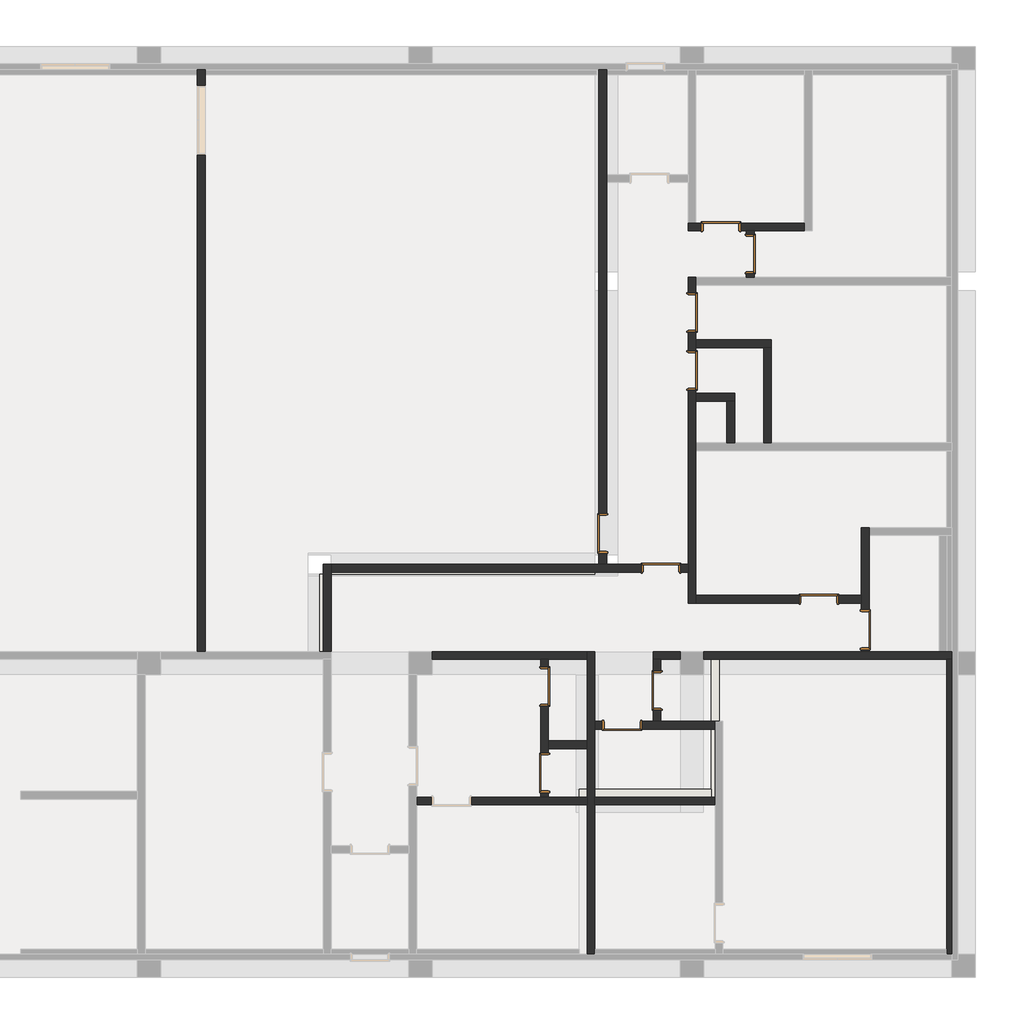
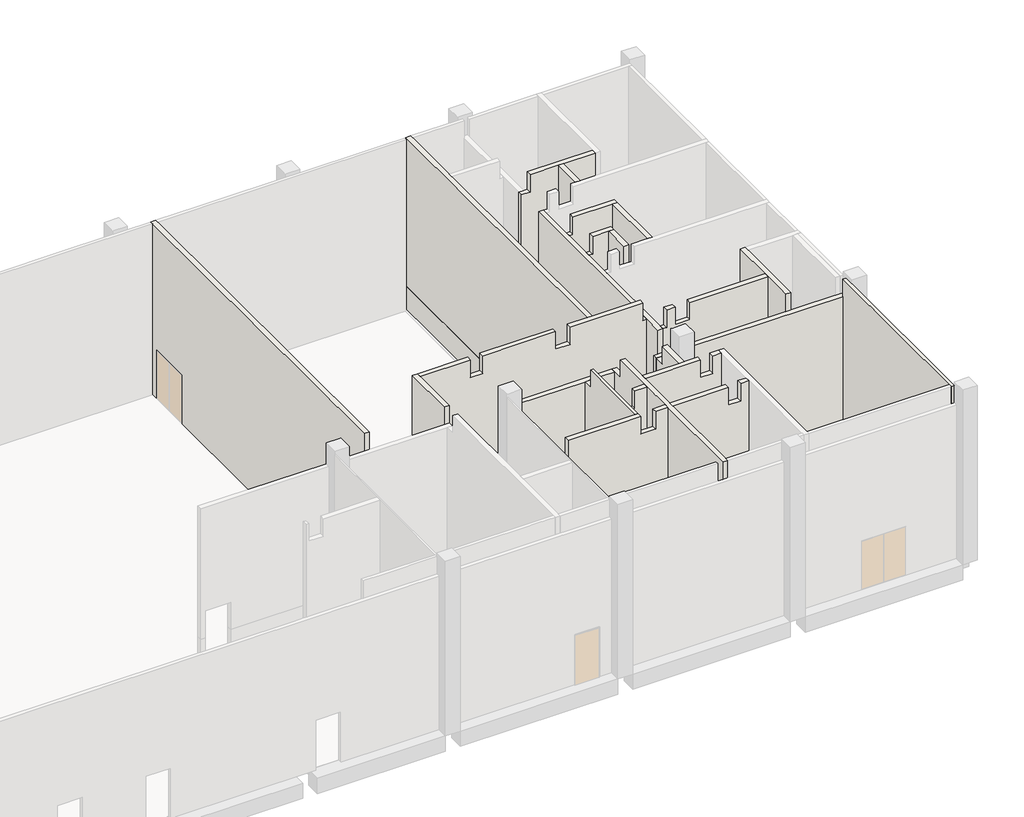
# One storey, part 2 of 4: 29 walls, 12 doors.
"""IFC4 building model written with IfcOpenShell, lengths in millimetres."""

import ifcopenshell
import ifcopenshell.guid

model = None  # the IFC model being written
_history = None  # IfcOwnerHistory: only IFC2X3 demands one
_inside = {}  # id of a spatial element -> (the spatial element, [elements in it])
_under = {}  # id of a project, library or spatial element -> (it, [spatial elements below it])
_declared = {}  # id of a project -> (the project, [libraries it declares])
_typed = {}  # id of a type object -> (the type object, [elements of that type])
_made_of = {}  # id of a material, layer set ... -> (it, [elements and type objects made of it])


def new_model(schema):
    """Start an empty IFC model of exactly this schema.

    Asked for "IFC4X3", IfcOpenShell would pick the latest addendum, in which some entities
    have other attributes; the version numbers below select the first issue.
    IFC2X3 requires an IfcOwnerHistory on every rooted entity: one is made here for all.
    """
    global model, _history
    if schema == "IFC4X3":
        model = ifcopenshell.file(schema_version=(4, 3, 0, 0))
    else:
        model = ifcopenshell.file(schema=schema)
    _inside.clear()
    _under.clear()
    _declared.clear()
    _typed.clear()
    _made_of.clear()
    _history = None
    if model.schema == "IFC2X3":
        org = make("IfcOrganization", Name="unknown")
        user = make(
            "IfcPersonAndOrganization",
            ThePerson=make("IfcPerson", FamilyName="unknown"),
            TheOrganization=org,
        )
        app = make(
            "IfcApplication",
            ApplicationDeveloper=org,
            Version="unknown",
            ApplicationFullName="unknown",
            ApplicationIdentifier="unknown",
        )
        _history = make(
            "IfcOwnerHistory",
            OwningUser=user,
            OwningApplication=app,
            ChangeAction="ADDED",
            CreationDate=0,
        )
    return model


def make(cls, **values):
    """One entity of the class cls with the attributes given. An attribute that is None is left unset."""
    return model.create_entity(
        cls, **{name: value for name, value in values.items() if value is not None}
    )


def rooted(cls, **values):
    """An entity with a GlobalId (a new one), such as an element, a storey or a relation."""
    return make(cls, GlobalId=ifcopenshell.guid.new(), OwnerHistory=_history, **values)


def si_unit(unit_type, name, prefix=None):
    """IfcSIUnit, for example si_unit("LENGTHUNIT", "METRE", prefix="MILLI")."""
    return make("IfcSIUnit", UnitType=unit_type, Prefix=prefix, Name=name)


def assignment(units):
    """IfcUnitAssignment: the units of a project."""
    return None if units is None else make("IfcUnitAssignment", Units=units)


def point(xyz):
    """IfcCartesianPoint."""
    return None if xyz is None else make("IfcCartesianPoint", Coordinates=xyz)


def direction(xyz):
    """IfcDirection."""
    return None if xyz is None else make("IfcDirection", DirectionRatios=xyz)


def frame(location, z_axis=None, x_axis=None):
    """IfcAxis2Placement3D, a coordinate frame: its origin and axes. An axis left out is left unset."""
    return make(
        "IfcAxis2Placement3D",
        Location=point(location),
        Axis=direction(z_axis),
        RefDirection=direction(x_axis),
    )


def origin():
    """The frame at (0, 0, 0) with its axes left unset."""
    return frame((0.0, 0.0, 0.0))


def origin_with_axes():
    """The frame at (0, 0, 0) with the z axis (0, 0, 1) and the x axis (1, 0, 0) written out."""
    return frame((0.0, 0.0, 0.0), z_axis=(0.0, 0.0, 1.0), x_axis=(1.0, 0.0, 0.0))


def place(relative_to, where):
    """IfcLocalPlacement: puts the frame where relative to a parent placement (None: the world)."""
    return make(
        "IfcLocalPlacement", PlacementRelTo=relative_to, RelativePlacement=where
    )


def context(
    kind, dimensions, precision=None, world=None, true_north=None, identifier=None
):
    """IfcGeometricRepresentationContext, for example the 3D "Model" context."""
    return make(
        "IfcGeometricRepresentationContext",
        ContextIdentifier=identifier,
        ContextType=kind,
        CoordinateSpaceDimension=dimensions,
        Precision=precision,
        WorldCoordinateSystem=world,
        TrueNorth=true_north,
    )


def project(units=None, contexts=None):
    """IfcProject with its units and contexts."""
    return rooted(
        "IfcProject",
        Name="project",
        RepresentationContexts=contexts,
        UnitsInContext=assignment(units),
    )


def spatial(cls, under=None, at=None, **own):
    """A site, building, storey or space (cls), placed at a placement, below another one or the project."""
    s = rooted(cls, ObjectPlacement=at, **own)
    if under is not None:
        _under.setdefault(under.id(), (under, []))[1].append(s)
    return s


def polyline(points):
    """IfcPolyline through the points."""
    return make("IfcPolyline", Points=[point(p) for p in points])


def outline(outer, holes=None, kind="AREA"):
    """IfcArbitraryClosedProfileDef: a profile drawn as a closed curve; with holes, ...WithVoids."""
    if holes is None:
        return make("IfcArbitraryClosedProfileDef", ProfileType=kind, OuterCurve=outer)
    return make(
        "IfcArbitraryProfileDefWithVoids",
        ProfileType=kind,
        OuterCurve=outer,
        InnerCurves=holes,
    )


def extrude(swept, where, along, depth):
    """IfcExtrudedAreaSolid: the profile swept, set in the frame where, extruded along a direction by depth."""
    return make(
        "IfcExtrudedAreaSolid",
        SweptArea=swept,
        Position=where,
        ExtrudedDirection=direction(along),
        Depth=depth,
    )


def faces_of(points, faces, orient=None, outer=None):
    """IfcFace entities. A face is a list of loops; a loop is a list of indices into points, from 0.

    orient and outer hold one flag for each loop. By default every Orientation is true, the
    first loop of a face is its IfcFaceOuterBound and the others are IfcFaceBound.
    """
    made = []
    for i, loops in enumerate(faces):
        bounds = []
        for j, loop in enumerate(loops):
            is_outer = j == 0 if outer is None else outer[i][j]
            bounds.append(
                make(
                    "IfcFaceOuterBound" if is_outer else "IfcFaceBound",
                    Bound=make("IfcPolyLoop", Polygon=[points[k] for k in loop]),
                    Orientation=True if orient is None else orient[i][j],
                )
            )
        made.append(make("IfcFace", Bounds=bounds))
    return made


def faceted_brep(points, faces, orient=None, outer=None, voids=None):
    """IfcFacetedBrep: a solid bounded by flat faces; with voids (closed shells), ...WithVoids."""
    shared = [point(p) for p in points]
    hull = make("IfcClosedShell", CfsFaces=faces_of(shared, faces, orient, outer))
    if voids is None:
        return make("IfcFacetedBrep", Outer=hull)
    return make(
        "IfcFacetedBrepWithVoids",
        Outer=hull,
        Voids=[
            make(cls, CfsFaces=faces_of(shared, fs, o, b)) for cls, fs, o, b in voids
        ],
    )


def shape(context_of_items, identifier, shape_type, items):
    """IfcShapeRepresentation: the items that make up one representation, for example the "Body"."""
    return make(
        "IfcShapeRepresentation",
        ContextOfItems=context_of_items,
        RepresentationIdentifier=identifier,
        RepresentationType=shape_type,
        Items=items,
    )


def source(mapping_origin, context_of_items, identifier, shape_type, items):
    """IfcRepresentationMap: a shape defined once, which mapped items show again and again."""
    return make(
        "IfcRepresentationMap",
        MappingOrigin=mapping_origin,
        MappedRepresentation=shape(context_of_items, identifier, shape_type, items),
    )


def transform(
    local_origin,
    x_axis=None,
    y_axis=None,
    z_axis=None,
    scale=None,
    scale2=None,
    scale3=None,
    uniform=True,
):
    """IfcCartesianTransformationOperator3D, or its non-uniform kind. x_axis, y_axis, z_axis: its Axis1, 2, 3."""
    if uniform:
        return make(
            "IfcCartesianTransformationOperator3D",
            Axis1=direction(x_axis),
            Axis2=direction(y_axis),
            LocalOrigin=point(local_origin),
            Scale=scale,
            Axis3=direction(z_axis),
        )
    return make(
        "IfcCartesianTransformationOperator3DnonUniform",
        Axis1=direction(x_axis),
        Axis2=direction(y_axis),
        LocalOrigin=point(local_origin),
        Scale=scale,
        Axis3=direction(z_axis),
        Scale2=scale2,
        Scale3=scale3,
    )


def mapped(mapping_source, mapping_target):
    """IfcMappedItem: shows the shape of a source again, moved by a transform."""
    return make(
        "IfcMappedItem", MappingSource=mapping_source, MappingTarget=mapping_target
    )


def made_of(thing, what):
    """Note that an element or type object is made of a material, layer set ...; save() writes the relation."""
    if what is not None:
        _made_of.setdefault(what.id(), (what, []))[1].append(thing)
    return thing


def element(
    cls,
    number,
    at=None,
    inside=None,
    cuts=None,
    type_object=None,
    material=None,
    context=None,
    identifier="Body",
    shape_type=None,
    held_by="IfcProductDefinitionShape",
    body=None,
    shapes=None,
    **own,
):
    """One element of the class cls, such as IfcWall. Its Tag is "e" and its number.

    at: its placement. inside: the storey or other place that contains it. cuts: it is an
    opening in that element (IfcRelVoidsElement). A single representation is given by context,
    identifier, shape_type and body (its items); several are given by shapes. held_by: the class
    of the entity that holds the representations. save() writes the other relations.
    """
    e = rooted(cls, Tag="e%d" % number, ObjectPlacement=at, **own)
    if body is not None:
        shapes = [shape(context, identifier, shape_type, body)]
    if shapes is not None:
        e.Representation = make(held_by, Representations=shapes)
    if inside is not None:
        _inside.setdefault(inside.id(), (inside, []))[1].append(e)
    if cuts is not None:
        rooted(
            "IfcRelVoidsElement", RelatingBuildingElement=cuts, RelatedOpeningElement=e
        )
    if type_object is not None:
        _typed.setdefault(type_object.id(), (type_object, []))[1].append(e)
    return made_of(e, material)


def aggregate(whole, parts):
    """IfcRelAggregates: a whole, such as a stair, and the parts it consists of."""
    return rooted("IfcRelAggregates", RelatingObject=whole, RelatedObjects=parts)


def save(model, path):
    """Write the relations noted so far, then the file.

    IfcRelAggregates (storeys below a building ...), IfcRelContainedInSpatialStructure (elements
    in a storey), IfcRelDefinesByType, IfcRelAssociatesMaterial and IfcRelDeclares: one each for
    every whole, place, type object, material and project.
    """
    for whole, parts in _under.values():
        aggregate(whole, parts)
    for where, things in _inside.values():
        rooted(
            "IfcRelContainedInSpatialStructure",
            RelatedElements=things,
            RelatingStructure=where,
        )
    for kind, things in _typed.values():
        rooted("IfcRelDefinesByType", RelatedObjects=things, RelatingType=kind)
    for what, things in _made_of.values():
        rooted("IfcRelAssociatesMaterial", RelatedObjects=things, RelatingMaterial=what)
    for by, libraries in _declared.values():
        rooted("IfcRelDeclares", RelatingContext=by, RelatedDefinitions=libraries)
    model.write(path)


def single_door_steel_f73fbc53(model_context):
    return source(origin(), model_context, "Body", "SolidModel", [
        extrude(outline(polyline([(480.0, -130.0), (-480.0, -130.0), (-480.0, -95.0), (480.0, -95.0), (480.0, -130.0)])), origin_with_axes(), (0.0, 0.0, 1.0), 2130.0),
        faceted_brep([(480.0, -130.0, 0.0), (480.0, -95.0, 0.0), (460.0, -95.0, 0.0), (460.0, 95.0, 0.0), (480.0, 95.0, 0.0), (480.0, 130.0, 0.0), (510.0, 130.0, 0.0), (510.0, -130.0, 0.0), (510.0, -130.0, 2160.0), (-510.0, -130.0, 2160.0), (-510.0, -130.0, 0.0), (-480.0, -130.0, 0.0), (-480.0, -130.0, 2130.0), (480.0, -130.0, 2130.0), (510.0, 130.0, 2160.0), (480.0, 130.0, 2130.0), (-480.0, 130.0, 2130.0), (-480.0, 130.0, 0.0), (-510.0, 130.0, 0.0), (-510.0, 130.0, 2160.0), (480.0, 95.0, 2130.0), (460.0, 95.0, 2110.0), (-460.0, 95.0, 2110.0), (-460.0, 95.0, 0.0), (-480.0, 95.0, 0.0), (-480.0, 95.0, 2130.0), (460.0, -95.0, 2110.0), (480.0, -95.0, 2130.0), (-480.0, -95.0, 2130.0), (-480.0, -95.0, 0.0), (-460.0, -95.0, 0.0), (-460.0, -95.0, 2110.0)], [[[0, 1, 2, 3, 4, 5, 6, 7]], [[7, 8, 9, 10, 11, 12, 13, 0]], [[6, 14, 8, 7]], [[5, 15, 16, 17, 18, 19, 14, 6]], [[4, 20, 15, 5]], [[3, 21, 22, 23, 24, 25, 20, 4]], [[2, 26, 21, 3]], [[1, 27, 28, 29, 30, 31, 26, 2]], [[0, 13, 27, 1]], [[12, 11, 29, 28]], [[11, 10, 18, 17, 24, 23, 30, 29]], [[19, 18, 10, 9]], [[25, 24, 17, 16]], [[31, 30, 23, 22]], [[14, 19, 9, 8]], [[20, 25, 16, 15]], [[26, 31, 22, 21]], [[13, 12, 28, 27]]]),
    ])


def single_door_steel_4bf023c6(model_context):
    return source(origin(), model_context, "Body", "SolidModel", [
        extrude(outline(polyline([(480.0, 130.0), (480.0, 95.0), (-480.0, 95.0), (-480.0, 130.0), (480.0, 130.0)])), origin_with_axes(), (0.0, 0.0, 1.0), 2130.0),
        faceted_brep([(480.0, 130.0, 0.0), (510.0, 130.0, 0.0), (510.0, -130.0, 0.0), (480.0, -130.0, 0.0), (480.0, -95.0, 0.0), (460.0, -95.0, 0.0), (460.0, 95.0, 0.0), (480.0, 95.0, 0.0), (480.0, 130.0, 2130.0), (-480.0, 130.0, 2130.0), (-480.0, 130.0, 0.0), (-510.0, 130.0, 0.0), (-510.0, 130.0, 2160.0), (510.0, 130.0, 2160.0), (510.0, -130.0, 2160.0), (-510.0, -130.0, 2160.0), (-510.0, -130.0, 0.0), (-480.0, -130.0, 0.0), (-480.0, -130.0, 2130.0), (480.0, -130.0, 2130.0), (480.0, -95.0, 2130.0), (-480.0, -95.0, 2130.0), (-480.0, -95.0, 0.0), (-460.0, -95.0, 0.0), (-460.0, -95.0, 2110.0), (460.0, -95.0, 2110.0), (460.0, 95.0, 2110.0), (-460.0, 95.0, 2110.0), (-460.0, 95.0, 0.0), (-480.0, 95.0, 0.0), (-480.0, 95.0, 2130.0), (480.0, 95.0, 2130.0)], [[[0, 1, 2, 3, 4, 5, 6, 7]], [[1, 0, 8, 9, 10, 11, 12, 13]], [[2, 1, 13, 14]], [[3, 2, 14, 15, 16, 17, 18, 19]], [[4, 3, 19, 20]], [[5, 4, 20, 21, 22, 23, 24, 25]], [[6, 5, 25, 26]], [[7, 6, 26, 27, 28, 29, 30, 31]], [[0, 7, 31, 8]], [[9, 30, 29, 10]], [[10, 29, 28, 23, 22, 17, 16, 11]], [[15, 12, 11, 16]], [[21, 18, 17, 22]], [[27, 24, 23, 28]], [[14, 13, 12, 15]], [[20, 19, 18, 21]], [[26, 25, 24, 27]], [[8, 31, 30, 9]]]),
    ])


model = new_model("IFC4")

# Units and contexts
model_context = context("Model", 3, world=origin())
ifc_project = project(units=[si_unit("LENGTHUNIT", "METRE", prefix="MILLI")], contexts=[model_context])

# Site, building, storey
site = spatial("IfcSite", under=ifc_project)
building = spatial("IfcBuilding", under=site)
storey = spatial("IfcBuildingStorey", under=building, Name="TOC(GF)", Elevation=97049.9618634)

# Doors
placement = place(None, origin())
single_door_steel_shape = single_door_steel_f73fbc53(model_context)
element("IfcDoor", 1, ObjectType="Single Door_Steel : H_DR_AR B12_Door_Single FSD 01", at=placement, inside=storey, context=model_context, shape_type="MappedRepresentation", body=[
    mapped(single_door_steel_shape, transform((47500.0, -1150.0, 97049.9618634), x_axis=(0.0, 1.0, 0.0), y_axis=(-1.0, 0.0, 0.0), z_axis=(0.0, 0.0, 1.0))),
])
element("IfcDoor", 2, ObjectType="Single Door_Steel : H_DR_AR B12_Door_Single FSD 01", at=placement, inside=storey, context=model_context, shape_type="MappedRepresentation", body=[
    mapped(single_door_steel_shape, transform((45200.0, -9250.0, 97049.9618634), x_axis=(-1.0, 0.0, 0.0), y_axis=(0.0, -1.0, 0.0), z_axis=(0.0, 0.0, 1.0))),
])
element("IfcDoor", 3, ObjectType="Single Door_Steel : H_DR_AR B12_Door_Single FSD 01", at=placement, inside=storey, context=model_context, shape_type="MappedRepresentation", body=[
    mapped(single_door_steel_shape, transform((50470.0, -10836.4720793, 97049.9618634), x_axis=(0.0, 1.0, 0.0), y_axis=(-1.0, 0.0, 0.0), z_axis=(0.0, 0.0, 1.0))),
])
element("IfcDoor", 4, ObjectType="Single Door_Steel : H_DR_AR B12_Door_Single FSD 01", at=placement, inside=storey, context=model_context, shape_type="MappedRepresentation", body=[
    mapped(single_door_steel_shape, transform((44201.4300122, -13300.0, 97049.9618634), x_axis=(1.0, 0.0, 0.0), y_axis=(0.0, 1.0, 0.0), z_axis=(0.0, 0.0, 1.0))),
])
single_door_steel_2_shape = single_door_steel_4bf023c6(model_context)
element("IfcDoor", 5, ObjectType="Single Door_Steel : H_DR_AR B12_Door_Single FSD 01", at=placement, inside=storey, context=model_context, shape_type="MappedRepresentation", body=[
    mapped(single_door_steel_2_shape, transform((46750.0, -450.0, 97049.9618634), x_axis=(1.0, 0.0, 0.0), y_axis=(0.0, 1.0, 0.0), z_axis=(0.0, 0.0, 1.0))),
])
element("IfcDoor", 6, ObjectType="Single Door_Steel : H_DR_AR B12_Door_Single FSD 01", at=placement, inside=storey, context=model_context, shape_type="MappedRepresentation", body=[
    mapped(single_door_steel_2_shape, transform((46000.0, -2657.5, 97049.9618634), x_axis=(0.0, -1.0, 0.0), y_axis=(1.0, 0.0, 0.0), z_axis=(0.0, 0.0, 1.0))),
])
element("IfcDoor", 7, ObjectType="Single Door_Steel : H_DR_AR B12_Door_Single FSD 01", at=placement, inside=storey, context=model_context, shape_type="MappedRepresentation", body=[
    mapped(single_door_steel_2_shape, transform((46000.0, -4155.0, 97049.9618634), x_axis=(0.0, -1.0, 0.0), y_axis=(1.0, 0.0, 0.0), z_axis=(0.0, 0.0, 1.0))),
])
element("IfcDoor", 8, ObjectType="Single Door_Steel : H_DR_AR B12_Door_Single FSD 01", at=placement, inside=storey, context=model_context, shape_type="MappedRepresentation", body=[
    mapped(single_door_steel_2_shape, transform((43700.0, -8350.0, 97049.9618634), x_axis=(0.0, 1.0, 0.0), y_axis=(-1.0, 0.0, 0.0), z_axis=(0.0, 0.0, 1.0))),
])
element("IfcDoor", 9, ObjectType="Single Door_Steel : H_DR_AR B12_Door_Single FSD 01", at=placement, inside=storey, context=model_context, shape_type="MappedRepresentation", body=[
    mapped(single_door_steel_2_shape, transform((49270.0, -10050.0, 97049.9618634), x_axis=(1.0, 0.0, 0.0), y_axis=(0.0, 1.0, 0.0), z_axis=(0.0, 0.0, 1.0))),
])
element("IfcDoor", 10, ObjectType="Single Door_Steel : H_DR_AR B12_Door_Single FSD 01", at=placement, inside=storey, context=model_context, shape_type="MappedRepresentation", body=[
    mapped(single_door_steel_2_shape, transform((45100.0, -12400.0, 97049.9618634), x_axis=(0.0, 1.0, 0.0), y_axis=(-1.0, 0.0, 0.0), z_axis=(0.0, 0.0, 1.0))),
])
element("IfcDoor", 11, ObjectType="Single Door_Steel : H_DR_AR B12_Door_Single FSD 01", at=placement, inside=storey, context=model_context, shape_type="MappedRepresentation", body=[
    mapped(single_door_steel_2_shape, transform((42200.0, -12300.0, 97049.9618634), x_axis=(0.0, -1.0, 0.0), y_axis=(1.0, 0.0, 0.0), z_axis=(0.0, 0.0, 1.0))),
])
element("IfcDoor", 12, ObjectType="Single Door_Steel : H_DR_AR B12_Door_Single FSD 01", at=placement, inside=storey, context=model_context, shape_type="MappedRepresentation", body=[
    mapped(single_door_steel_2_shape, transform((42200.0, -14524.618743, 97049.9618634), x_axis=(0.0, 1.0, 0.0), y_axis=(-1.0, 0.0, 0.0), z_axis=(0.0, 0.0, 1.0))),
])

# Walls
element("IfcWall", 13, ObjectType="H_WA_AR_B02_Ext Wall_RC_T200_W2", at=placement, inside=storey, context=model_context, shape_type="Brep", body=[
    faceted_brep([(36700.0, -9200.0, 97049.9618634), (36700.0, -9200.0, 98049.9618634), (43500.0, -9200.0, 98049.9618634), (43500.0, -9200.0, 97049.9618634), (36700.0, -9400.0, 98049.9618634), (36700.0, -9400.0, 97049.9618634), (43500.0, -9400.0, 97049.9618634), (43500.0, -9400.0, 98049.9618634), (36700.0, -9350.0, 98049.9618634)], [[[0, 1, 2, 3]], [[4, 5, 6, 7]], [[5, 0, 3, 6]], [[1, 8, 4, 7, 2]], [[1, 0, 5, 4, 8]], [[3, 2, 7, 6]]]),
])
element("IfcWall", 14, ObjectType="H_WA_AR_B02_Ext Wall_RC_T200_W2", at=placement, inside=storey, context=model_context, shape_type="Brep", body=[
    faceted_brep([(36400.0, -9400.0, 97049.9618634), (36400.0, -11400.0, 97049.9618634), (36400.0, -11600.0, 97049.9618634), (36400.0, -11600.0, 98049.9618634), (36400.0, -11400.0, 98049.9618634), (36400.0, -9400.0, 98049.9618634), (36600.0, -9400.0, 97049.9618634), (36600.0, -9400.0, 98049.9618634), (36600.0, -11400.0, 98049.9618634), (36600.0, -11600.0, 98049.9618634), (36600.0, -11600.0, 97049.9618634), (36600.0, -11400.0, 97049.9618634), (36500.0, -11600.0, 97049.9618634)], [[[0, 1, 2, 3, 4, 5]], [[6, 7, 8, 9, 10, 11]], [[2, 1, 0, 6, 11, 10, 12]], [[5, 4, 3, 9, 8, 7]], [[0, 5, 7, 6]], [[3, 2, 12, 10, 9]]]),
])
element("IfcWall", 15, ObjectType="H_WA_AR_B02_Ext Wall_RC_T200_W2", at=placement, inside=storey, context=model_context, shape_type="Brep", body=[
    faceted_brep([(43800.0, -8900.0, 98049.9618634), (43800.0, -8900.0, 97049.9618634), (43800.0, -8860.0, 97049.9618634), (43800.0, -8860.0, 98049.9618634), (43600.0, -8900.0, 97049.9618634), (43600.0, -8900.0, 98049.9618634), (43600.0, -8860.0, 98049.9618634), (43600.0, -8860.0, 97049.9618634)], [[[0, 1, 2, 3]], [[4, 5, 6, 7]], [[1, 4, 7, 2]], [[5, 0, 3, 6]], [[1, 0, 5, 4]], [[3, 2, 7, 6]]]),
    faceted_brep([(43800.0, -7840.0, 98049.9618634), (43800.0, -7840.0, 97049.9618634), (43800.0, -2100.0, 97049.9618634), (43800.0, -2100.0, 98049.9618634), (43600.0, -7840.0, 97049.9618634), (43600.0, -7840.0, 98049.9618634), (43600.0, -2100.0, 98049.9618634), (43600.0, -2100.0, 97049.9618634)], [[[0, 1, 2, 3]], [[4, 5, 6, 7]], [[1, 4, 7, 2]], [[5, 0, 3, 6]], [[3, 2, 7, 6]], [[1, 0, 5, 4]]]),
    faceted_brep([(43800.0, 3600.0, 97049.9618634), (43800.0, 3600.0, 98049.9618634), (43800.0, -1600.0, 98049.9618634), (43800.0, -1600.0, 97049.9618634), (43800.0, 700.0, 97049.9618634), (43800.0, 900.0, 97049.9618634), (43800.0, 3474.0, 97049.9618634), (43600.0, 3600.0, 98049.9618634), (43600.0, 3600.0, 97049.9618634), (43600.0, -1600.0, 97049.9618634), (43600.0, -1600.0, 98049.9618634)], [[[0, 1, 2, 3, 4, 5, 6]], [[7, 8, 9, 10]], [[8, 0, 6, 5, 4, 3, 9]], [[1, 7, 10, 2]], [[1, 0, 8, 7]], [[3, 2, 10, 9]]]),
])
element("IfcWall", 16, ObjectType="H_WA_AR_B02_Ext Wall_RC_T200_W2", at=placement, inside=storey, context=model_context, shape_type="Brep", body=[
    faceted_brep([(46300.0, -11600.0, 97049.9618634), (46500.0, -11600.0, 97049.9618634), (46700.0, -11600.0, 97049.9618634), (52574.0, -11600.0, 97049.9618634), (52700.0, -11600.0, 97049.9618634), (52700.0, -11600.0, 98049.9618634), (52574.0, -11600.0, 98049.9618634), (46700.0, -11600.0, 98049.9618634), (46500.0, -11600.0, 98049.9618634), (46300.0, -11600.0, 98049.9618634), (46300.0, -11400.0, 97049.9618634), (46300.0, -11400.0, 98049.9618634), (52574.0, -11400.0, 98049.9618634), (52700.0, -11400.0, 98049.9618634), (52700.0, -11400.0, 97049.9618634), (52574.0, -11400.0, 97049.9618634), (52374.0, -11400.0, 97049.9618634), (50570.0, -11400.0, 97049.9618634), (50370.0, -11400.0, 97049.9618634)], [[[0, 1, 2, 3, 4, 5, 6, 7, 8, 9]], [[10, 11, 12, 13, 14, 15, 16, 17, 18]], [[4, 3, 2, 1, 0, 10, 18, 17, 16, 15, 14]], [[9, 8, 7, 6, 5, 13, 12, 11]], [[0, 9, 11, 10]], [[5, 4, 14, 13]]]),
])
element("IfcWall", 17, ObjectType="H_WA_AR_B02_Ext Wall_RC_T200_W2", at=placement, inside=storey, context=model_context, shape_type="Brep", body=[
    faceted_brep([(46500.0, -11600.0, 97049.9618634), (46500.0, -13200.0, 97049.9618634), (46500.0, -13400.0, 97049.9618634), (46500.0, -14950.0, 97049.9618634), (46500.0, -15150.0, 97049.9618634), (46500.0, -15150.0, 98049.9618634), (46500.0, -14950.0, 98049.9618634), (46500.0, -13400.0, 98049.9618634), (46500.0, -13200.0, 98049.9618634), (46500.0, -11600.0, 98049.9618634), (46700.0, -11600.0, 97049.9618634), (46700.0, -11600.0, 98049.9618634), (46700.0, -13200.0, 98049.9618634), (46700.0, -15150.0, 98049.9618634), (46700.0, -15150.0, 97049.9618634), (46700.0, -13200.0, 97049.9618634), (46600.0, -15150.0, 97049.9618634), (46600.0, -15150.0, 98049.9618634)], [[[0, 1, 2, 3, 4, 5, 6, 7, 8, 9]], [[10, 11, 12, 13, 14, 15]], [[4, 3, 2, 1, 0, 10, 15, 14, 16]], [[9, 8, 7, 6, 5, 17, 13, 12, 11]], [[0, 9, 11, 10]], [[5, 4, 16, 14, 13, 17]]]),
])
element("IfcWall", 18, ObjectType="H_WA_AR_B02_Ext Wall_RC_T200_W2", at=placement, inside=storey, context=model_context, shape_type="Brep", body=[
    faceted_brep([(46500.0, -14950.0, 97049.9618634), (43500.0, -14950.0, 97049.9618634), (43300.0, -14950.0, 97049.9618634), (43100.0, -14950.0, 97049.9618634), (43100.0, -14950.0, 98049.9618634), (43300.0, -14950.0, 98049.9618634), (43500.0, -14950.0, 98049.9618634), (46500.0, -14950.0, 98049.9618634), (46500.0, -15150.0, 97049.9618634), (46500.0, -15150.0, 98049.9618634), (43500.0, -15150.0, 98049.9618634), (43300.0, -15150.0, 98049.9618634), (43100.0, -15150.0, 98049.9618634), (43100.0, -15150.0, 97049.9618634), (43300.0, -15150.0, 97049.9618634), (43500.0, -15150.0, 97049.9618634)], [[[0, 1, 2, 3, 4, 5, 6, 7]], [[8, 9, 10, 11, 12, 13, 14, 15]], [[3, 2, 1, 0, 8, 15, 14, 13]], [[7, 6, 5, 4, 12, 11, 10, 9]], [[0, 7, 9, 8]], [[4, 3, 13, 12]]]),
])
element("IfcWall", 19, ObjectType="H_WA_AR B02_Int Wall MA_IW1 T200", at=placement, inside=storey, context=model_context, shape_type="Brep", body=[
    faceted_brep([(36700.0, -11400.0, 97049.9618634), (36700.0, -9400.0, 97049.9618634), (36700.0, -9400.0, 98049.9618634), (36700.0, -9350.0, 98049.9618634), (36700.0, -9200.0, 98049.9618634), (36700.0, -9150.0, 98049.9618634), (36700.0, -9150.0, 104400.0), (36700.0, -9350.0, 104400.0), (36700.0, -11400.0, 104400.0), (36700.0, -11400.0, 103650.0), (36700.0, -11400.0, 98049.9618634), (36500.0, -11400.0, 104400.0), (36500.0, -9150.0, 104400.0), (36500.0, -9150.0, 98049.9618634), (36500.0, -11400.0, 98049.9618634), (36600.0, -11400.0, 97049.9618634), (36600.0, -9400.0, 97049.9618634), (36600.0, -9400.0, 98049.9618634), (36600.0, -11400.0, 98049.9618634)], [[[0, 1, 2, 3, 4, 5, 6, 7, 8, 9, 10]], [[11, 12, 13, 14]], [[1, 0, 15, 16]], [[8, 7, 6, 12, 11]], [[5, 4, 3, 2, 17, 18, 14, 13]], [[2, 1, 16, 17]], [[5, 13, 12, 6]], [[0, 10, 9, 8, 11, 14, 18, 15]], [[18, 17, 16, 15]]]),
])
element("IfcWall", 20, ObjectType="H_WA_AR B02_Int Wall MA_IW1 T200", at=placement, inside=storey, context=model_context, shape_type="Brep", body=[
    faceted_brep([(38750.0, -9350.0, 104400.0), (36700.0, -9350.0, 104400.0), (36700.0, -9350.0, 98049.9618634), (44100.0, -9350.0, 98049.9618634), (44100.0, -9350.0, 97049.9618634), (44690.0, -9350.0, 97049.9618634), (44690.0, -9350.0, 99209.9618634), (45710.0, -9350.0, 99209.9618634), (45710.0, -9350.0, 97049.9618634), (45900.0, -9350.0, 97049.9618634), (45900.0, -9350.0, 103650.0), (45750.0, -9350.0, 103650.0), (45750.0, -9350.0, 104400.0), (42800.0, -9350.0, 104400.0), (42800.0, -9350.0, 103650.0), (42200.0, -9350.0, 103650.0), (42200.0, -9350.0, 104400.0), (39250.0, -9350.0, 104400.0), (39250.0, -9350.0, 103650.0), (38750.0, -9350.0, 103650.0), (36700.0, -9150.0, 104400.0), (38750.0, -9150.0, 104400.0), (38750.0, -9150.0, 103650.0), (39250.0, -9150.0, 103650.0), (39250.0, -9150.0, 104400.0), (42200.0, -9150.0, 104400.0), (42200.0, -9150.0, 103650.0), (42800.0, -9150.0, 103650.0), (42800.0, -9150.0, 104400.0), (43600.0, -9150.0, 104400.0), (43800.0, -9150.0, 104400.0), (45750.0, -9150.0, 104400.0), (45750.0, -9150.0, 103650.0), (45900.0, -9150.0, 103650.0), (45900.0, -9150.0, 97049.9618634), (45710.0, -9150.0, 97049.9618634), (45710.0, -9150.0, 99209.9618634), (44690.0, -9150.0, 99209.9618634), (44690.0, -9150.0, 97049.9618634), (44100.0, -9150.0, 97049.9618634), (44100.0, -9150.0, 98049.9618634), (43800.0, -9150.0, 98049.9618634), (43600.0, -9150.0, 98049.9618634), (43500.0, -9150.0, 98049.9618634), (43500.0, -9150.0, 97049.9618634), (36700.0, -9150.0, 97049.9618634), (36700.0, -9150.0, 98049.9618634), (36700.0, -9200.0, 97049.9618634), (43500.0, -9200.0, 97049.9618634), (36700.0, -9200.0, 98049.9618634), (43500.0, -9200.0, 98049.9618634)], [[[0, 1, 2, 3, 4, 5, 6, 7, 8, 9, 10, 11, 12, 13, 14, 15, 16, 17, 18, 19]], [[20, 21, 22, 23, 24, 25, 26, 27, 28, 29, 30, 31, 32, 33, 34, 35, 36, 37, 38, 39, 40, 41, 42, 43, 44, 45, 46]], [[34, 9, 8, 35]], [[47, 45, 44, 48]], [[38, 5, 4, 39]], [[9, 34, 33, 10]], [[1, 0, 21, 20]], [[24, 17, 16, 25]], [[12, 31, 30, 29, 28, 13]], [[19, 22, 21, 0]], [[22, 19, 18, 23]], [[23, 18, 17, 24]], [[11, 32, 31, 12]], [[32, 11, 10, 33]], [[15, 26, 25, 16]], [[26, 15, 14, 27]], [[27, 14, 13, 28]], [[2, 1, 20, 46, 45, 47, 49]], [[49, 47, 48, 50]], [[2, 49, 50, 43, 42, 41, 40, 3]], [[43, 50, 48, 44]], [[3, 40, 39, 4]], [[6, 5, 38, 37]], [[7, 6, 37, 36]], [[8, 7, 36, 35]]]),
])
element("IfcWall", 21, ObjectType="H_WA_AR B02_Int Wall MA_IW1 T200", at=placement, inside=storey, context=model_context, shape_type="Brep", body=[
    faceted_brep([(46100.0, -2147.5, 97049.9618634), (46100.0, -1950.0, 97049.9618634), (46100.0, -1750.0, 97049.9618634), (46100.0, -1750.0, 103650.0), (46100.0, -1950.0, 103650.0), (46100.0, -3365.0, 103650.0), (46100.0, -3565.0, 103650.0), (46100.0, -4745.0, 103650.0), (46100.0, -4945.0, 103650.0), (46100.0, -6015.0, 103650.0), (46100.0, -6215.0, 103650.0), (46100.0, -9950.0, 103650.0), (46100.0, -10150.0, 103650.0), (46100.0, -10150.0, 97049.9618634), (46100.0, -9950.0, 97049.9618634), (46100.0, -6215.0, 97049.9618634), (46100.0, -6015.0, 97049.9618634), (46100.0, -4945.0, 97049.9618634), (46100.0, -4745.0, 97049.9618634), (46100.0, -4665.0, 97049.9618634), (46100.0, -4665.0, 99209.9618634), (46100.0, -3645.0, 99209.9618634), (46100.0, -3645.0, 97049.9618634), (46100.0, -3565.0, 97049.9618634), (46100.0, -3365.0, 97049.9618634), (46100.0, -3167.5, 97049.9618634), (46100.0, -3167.5, 99209.9618634), (46100.0, -2147.5, 99209.9618634), (45900.0, -1750.0, 97049.9618634), (45900.0, -2147.5, 97049.9618634), (45900.0, -2147.5, 99209.9618634), (45900.0, -3167.5, 99209.9618634), (45900.0, -3167.5, 97049.9618634), (45900.0, -3645.0, 97049.9618634), (45900.0, -3645.0, 99209.9618634), (45900.0, -4665.0, 99209.9618634), (45900.0, -4665.0, 97049.9618634), (45900.0, -9150.0, 97049.9618634), (45900.0, -9350.0, 97049.9618634), (45900.0, -10150.0, 97049.9618634), (45900.0, -10150.0, 103650.0), (45900.0, -9350.0, 103650.0), (45900.0, -9150.0, 103650.0), (45900.0, -1750.0, 103650.0)], [[[0, 1, 2, 3, 4, 5, 6, 7, 8, 9, 10, 11, 12, 13, 14, 15, 16, 17, 18, 19, 20, 21, 22, 23, 24, 25, 26, 27]], [[28, 29, 30, 31, 32, 33, 34, 35, 36, 37, 38, 39, 40, 41, 42, 43]], [[13, 39, 38, 37, 36, 19, 18, 17, 16, 15, 14]], [[28, 2, 1, 0, 29]], [[32, 25, 24, 23, 22, 33]], [[39, 13, 12, 40]], [[12, 11, 10, 9, 8, 7, 6, 5, 4, 3, 43, 42, 41, 40]], [[2, 28, 43, 3]], [[31, 26, 25, 32]], [[26, 31, 30, 27]], [[27, 30, 29, 0]], [[35, 20, 19, 36]], [[20, 35, 34, 21]], [[21, 34, 33, 22]]]),
])
element("IfcWall", 22, ObjectType="H_WA_AR B02_Int Wall MA_IW1 T200", at=placement, inside=storey, context=model_context, shape_type="Brep", body=[
    faceted_brep([(43800.0, 3600.0, 104400.0), (43800.0, 900.0, 104400.0), (43800.0, 700.0, 104400.0), (43800.0, -9150.0, 104400.0), (43800.0, -9150.0, 98049.9618634), (43800.0, -8900.0, 98049.9618634), (43800.0, -8860.0, 98049.9618634), (43800.0, -8860.0, 99209.9618634), (43800.0, -7840.0, 99209.9618634), (43800.0, -7840.0, 98049.9618634), (43800.0, -2100.0, 98049.9618634), (43800.0, -1600.0, 98049.9618634), (43800.0, 3600.0, 98049.9618634), (43600.0, -9150.0, 104400.0), (43600.0, 3600.0, 104400.0), (43600.0, 3600.0, 98049.9618634), (43600.0, -1600.0, 98049.9618634), (43600.0, -2100.0, 98049.9618634), (43600.0, -7840.0, 98049.9618634), (43600.0, -7840.0, 99209.9618634), (43600.0, -8860.0, 99209.9618634), (43600.0, -8860.0, 98049.9618634), (43600.0, -8900.0, 98049.9618634), (43600.0, -9150.0, 98049.9618634)], [[[0, 1, 2, 3, 4, 5, 6, 7, 8, 9, 10, 11, 12]], [[13, 14, 15, 16, 17, 18, 19, 20, 21, 22, 23]], [[14, 0, 12, 15]], [[3, 2, 1, 0, 14, 13]], [[3, 13, 23, 4]], [[12, 11, 10, 9, 18, 17, 16, 15]], [[6, 5, 4, 23, 22, 21]], [[8, 19, 18, 9]], [[19, 8, 7, 20]], [[20, 7, 6, 21]]]),
])
element("IfcWall", 23, ObjectType="H_WA_AR B02_Int Wall MA_IW1 T200", at=placement, inside=storey, context=model_context, shape_type="Brep", body=[
    faceted_brep([(48900.0, -350.0, 104400.0), (48900.0, -350.0, 97049.9618634), (47260.0, -350.0, 97049.9618634), (47260.0, -350.0, 99209.9618634), (46240.0, -350.0, 99209.9618634), (46240.0, -350.0, 97049.9618634), (46100.0, -350.0, 97049.9618634), (45900.0, -350.0, 97049.9618634), (45900.0, -350.0, 103650.0), (46100.0, -350.0, 103650.0), (46250.0, -350.0, 103650.0), (46250.0, -350.0, 104400.0), (48900.0, -550.0, 97049.9618634), (48900.0, -550.0, 104400.0), (47600.0, -550.0, 104400.0), (47400.0, -550.0, 104400.0), (46250.0, -550.0, 104400.0), (46250.0, -550.0, 103650.0), (45900.0, -550.0, 103650.0), (45900.0, -550.0, 97049.9618634), (46240.0, -550.0, 97049.9618634), (46240.0, -550.0, 99209.9618634), (47260.0, -550.0, 99209.9618634), (47260.0, -550.0, 97049.9618634), (47400.0, -550.0, 97049.9618634), (47600.0, -550.0, 97049.9618634)], [[[0, 1, 2, 3, 4, 5, 6, 7, 8, 9, 10, 11]], [[12, 13, 14, 15, 16, 17, 18, 19, 20, 21, 22, 23, 24, 25]], [[1, 12, 25, 24, 23, 2]], [[19, 7, 6, 5, 20]], [[12, 1, 0, 13]], [[13, 0, 11, 16, 15, 14]], [[17, 10, 9, 8, 18]], [[10, 17, 16, 11]], [[7, 19, 18, 8]], [[22, 3, 2, 23]], [[3, 22, 21, 4]], [[4, 21, 20, 5]]]),
])
element("IfcWall", 24, ObjectType="H_WA_AR B02_Int Wall MA_IW1 T200", at=placement, inside=storey, context=model_context, shape_type="Brep", body=[
    faceted_brep([(48050.0, -3365.0, 97049.9618634), (46100.0, -3365.0, 97049.9618634), (46100.0, -3365.0, 103650.0), (46250.0, -3365.0, 103650.0), (46250.0, -3365.0, 104400.0), (48050.0, -3365.0, 104400.0), (46100.0, -3565.0, 97049.9618634), (47850.0, -3565.0, 97049.9618634), (48050.0, -3565.0, 97049.9618634), (48050.0, -3565.0, 104400.0), (47850.0, -3565.0, 104400.0), (46250.0, -3565.0, 104400.0), (46250.0, -3565.0, 103650.0), (46100.0, -3565.0, 103650.0)], [[[0, 1, 2, 3, 4, 5]], [[6, 7, 8, 9, 10, 11, 12, 13]], [[1, 0, 8, 7, 6]], [[1, 6, 13, 2]], [[8, 0, 5, 9]], [[9, 5, 4, 11, 10]], [[12, 3, 2, 13]], [[3, 12, 11, 4]]]),
])
element("IfcWall", 25, ObjectType="H_WA_AR B02_Int Wall MA_IW1 T200", at=placement, inside=storey, context=model_context, shape_type="SweptSolid", body=[
    extrude(outline(polyline([(47850.0, -6015.0), (47850.0, -3565.0), (48050.0, -3565.0), (48050.0, -6015.0), (47850.0, -6015.0)])), frame((0.0, 0.0, 97049.9618634), z_axis=(0.0, 0.0, 1.0), x_axis=(1.0, 0.0, 0.0)), (0.0, 0.0, 1.0), 7350.0381366),
])
element("IfcWall", 26, ObjectType="H_WA_AR B02_Int Wall MA_IW1 T200", at=placement, inside=storey, context=model_context, shape_type="SweptSolid", body=[
    extrude(outline(polyline([(-550.0, 97049.9618634), (-640.0, 97049.9618634), (-640.0, 99209.9618634), (-1660.0, 99209.9618634), (-1660.0, 97049.9618634), (-1750.0, 97049.9618634), (-1750.0, 104400.0), (-550.0, 104400.0), (-550.0, 97049.9618634)])), frame((47400.0, 0.0, 0.0), z_axis=(1.0, 0.0, 0.0), x_axis=(0.0, 1.0, 0.0)), (0.0, 0.0, 1.0), 200.0),
])
element("IfcWall", 27, ObjectType="H_WA_AR B02_Int Wall MA_IW1 T200", at=placement, inside=storey, context=model_context, shape_type="SweptSolid", body=[
    extrude(outline(polyline([(46300.0, -11400.0), (52700.0, -11400.0), (52700.0, -11600.0), (46300.0, -11600.0), (46300.0, -11400.0)])), frame((0.0, 0.0, 98049.9618634), z_axis=(0.0, 0.0, 1.0), x_axis=(1.0, 0.0, 0.0)), (0.0, 0.0, 1.0), 5600.0381366),
])
element("IfcWall", 28, ObjectType="H_WA_AR B02_Int Wall MA_IW1 T200", at=placement, inside=storey, context=model_context, shape_type="Brep", body=[
    faceted_brep([(45700.0, -11400.0, 97049.9618634), (45000.0, -11400.0, 97049.9618634), (45000.0, -11400.0, 103650.0), (45700.0, -11400.0, 103650.0), (45000.0, -11600.0, 97049.9618634), (45200.0, -11600.0, 97049.9618634), (45700.0, -11600.0, 97049.9618634), (45700.0, -11600.0, 103650.0), (45200.0, -11600.0, 103650.0), (45000.0, -11600.0, 103650.0)], [[[0, 1, 2, 3]], [[4, 5, 6, 7, 8, 9]], [[1, 0, 6, 5, 4]], [[6, 0, 3, 7]], [[1, 4, 9, 2]], [[3, 2, 9, 8, 7]]]),
])
element("IfcWall", 29, ObjectType="H_WA_AR B02_Int Wall MA_IW1 T200", at=placement, inside=storey, context=model_context, shape_type="Brep", body=[
    faceted_brep([(43500.0, -11400.0, 97049.9618634), (43500.0, -11400.0, 103650.0), (43500.0, -12000.0, 103650.0), (43500.0, -12000.0, 104400.0), (43500.0, -13200.0, 104400.0), (43500.0, -13400.0, 104400.0), (43500.0, -15150.0, 104400.0), (43500.0, -15350.0, 104400.0), (43500.0, -19200.0, 104400.0), (43500.0, -19200.0, 97049.9618634), (43500.0, -19074.0, 97049.9618634), (43500.0, -15350.0, 97049.9618634), (43500.0, -15150.0, 97049.9618634), (43500.0, -15150.0, 98049.9618634), (43500.0, -14950.0, 98049.9618634), (43500.0, -14950.0, 97049.9618634), (43500.0, -13400.0, 97049.9618634), (43500.0, -13200.0, 97049.9618634), (43300.0, -19200.0, 104400.0), (43300.0, -15350.0, 104400.0), (43300.0, -15150.0, 104400.0), (43300.0, -13899.2374861, 104400.0), (43300.0, -13699.2374861, 104400.0), (43300.0, -12000.0, 104400.0), (43300.0, -12000.0, 103650.0), (43300.0, -11600.0, 103650.0), (43300.0, -11400.0, 103650.0), (43300.0, -11400.0, 97049.9618634), (43300.0, -11600.0, 97049.9618634), (43300.0, -13699.2374861, 97049.9618634), (43300.0, -13899.2374861, 97049.9618634), (43300.0, -14950.0, 97049.9618634), (43300.0, -14950.0, 98049.9618634), (43300.0, -15150.0, 98049.9618634), (43300.0, -15150.0, 97049.9618634), (43300.0, -19200.0, 97049.9618634)], [[[0, 1, 2, 3, 4, 5, 6, 7, 8, 9, 10, 11, 12, 13, 14, 15, 16, 17]], [[18, 19, 20, 21, 22, 23, 24, 25, 26, 27, 28, 29, 30, 31, 32, 33, 34, 35]], [[27, 0, 17, 16, 15, 31, 30, 29, 28]], [[9, 35, 34, 12, 11, 10]], [[35, 9, 8, 18]], [[0, 27, 26, 1]], [[8, 7, 6, 5, 4, 3, 23, 22, 21, 20, 19, 18]], [[24, 2, 1, 26, 25]], [[2, 24, 23, 3]], [[14, 32, 31, 15]], [[33, 13, 12, 34]], [[32, 14, 13, 33]]]),
])
element("IfcWall", 30, ObjectType="H_WA_AR B02_Int Wall MA_IW1 T200", at=placement, inside=storey, context=model_context, shape_type="Brep", body=[
    faceted_brep([(43300.0, -11400.0, 97049.9618634), (39300.0, -11400.0, 97049.9618634), (39300.0, -11400.0, 103650.0), (43300.0, -11400.0, 103650.0), (39300.0, -11600.0, 97049.9618634), (42100.0, -11600.0, 97049.9618634), (42300.0, -11600.0, 97049.9618634), (43300.0, -11600.0, 97049.9618634), (43300.0, -11600.0, 103650.0), (42300.0, -11600.0, 103650.0), (42100.0, -11600.0, 103650.0), (39300.0, -11600.0, 103650.0)], [[[0, 1, 2, 3]], [[4, 5, 6, 7, 8, 9, 10, 11]], [[1, 0, 7, 6, 5, 4]], [[1, 4, 11, 2]], [[7, 0, 3, 8]], [[3, 2, 11, 10, 9, 8]]]),
])
element("IfcWall", 31, ObjectType="H_WA_AR B02_Int Wall MA_IW1 T200", at=placement, inside=storey, context=model_context, shape_type="SweptSolid", body=[
    extrude(outline(polyline([(-13200.0, 97049.9618634), (-13200.0, 104400.0), (-12000.0, 104400.0), (-12000.0, 103650.0), (-11600.0, 103650.0), (-11600.0, 97049.9618634), (-11890.0, 97049.9618634), (-11890.0, 99209.9618634), (-12910.0, 99209.9618634), (-12910.0, 97049.9618634), (-13200.0, 97049.9618634)])), frame((45000.0, 0.0, 0.0), z_axis=(1.0, 0.0, 0.0), x_axis=(0.0, 1.0, 0.0)), (0.0, 0.0, 1.0), 200.0),
])
element("IfcWall", 32, ObjectType="H_WA_AR B02_Int Wall MA_IW1 T200", at=placement, inside=storey, context=model_context, shape_type="Brep", body=[
    faceted_brep([(43500.0, -13200.0, 97049.9618634), (43500.0, -13200.0, 104400.0), (45000.0, -13200.0, 104400.0), (45200.0, -13200.0, 104400.0), (45750.0, -13200.0, 104400.0), (45750.0, -13200.0, 103650.0), (46250.0, -13200.0, 103650.0), (46250.0, -13200.0, 104400.0), (46600.0, -13200.0, 104400.0), (46600.0, -13200.0, 98049.9618634), (46500.0, -13200.0, 98049.9618634), (46500.0, -13200.0, 97049.9618634), (45200.0, -13200.0, 97049.9618634), (45000.0, -13200.0, 97049.9618634), (44711.4300122, -13200.0, 97049.9618634), (44711.4300122, -13200.0, 99209.9618634), (43691.4300122, -13200.0, 99209.9618634), (43691.4300122, -13200.0, 97049.9618634), (43500.0, -13400.0, 104400.0), (43500.0, -13400.0, 97049.9618634), (43691.4300122, -13400.0, 97049.9618634), (43691.4300122, -13400.0, 99209.9618634), (44711.4300122, -13400.0, 99209.9618634), (44711.4300122, -13400.0, 97049.9618634), (46500.0, -13400.0, 97049.9618634), (46500.0, -13400.0, 98049.9618634), (46600.0, -13400.0, 98049.9618634), (46600.0, -13400.0, 104400.0), (46250.0, -13400.0, 104400.0), (46250.0, -13400.0, 103650.0), (45750.0, -13400.0, 103650.0), (45750.0, -13400.0, 104400.0)], [[[0, 1, 2, 3, 4, 5, 6, 7, 8, 9, 10, 11, 12, 13, 14, 15, 16, 17]], [[18, 19, 20, 21, 22, 23, 24, 25, 26, 27, 28, 29, 30, 31]], [[19, 0, 17, 20]], [[23, 14, 13, 12, 11, 24]], [[8, 27, 26, 9]], [[0, 19, 18, 1]], [[27, 8, 7, 28]], [[1, 18, 31, 4, 3, 2]], [[30, 5, 4, 31]], [[5, 30, 29, 6]], [[6, 29, 28, 7]], [[10, 25, 24, 11]], [[25, 10, 9, 26]], [[15, 14, 23, 22]], [[16, 15, 22, 21]], [[17, 16, 21, 20]]]),
])
element("IfcWall", 33, ObjectType="H_WA_AR B02_Int Wall MA_IW1 T200", at=placement, inside=storey, context=model_context, shape_type="Brep", body=[
    faceted_brep([(38900.0, -15150.0, 97049.9618634), (38900.0, -15150.0, 103650.0), (39250.0, -15150.0, 103650.0), (39250.0, -15150.0, 104400.0), (42100.0, -15150.0, 104400.0), (42200.0, -15150.0, 104400.0), (42200.0, -15150.0, 103650.0), (42300.0, -15150.0, 103650.0), (42800.0, -15150.0, 103650.0), (42800.0, -15150.0, 104400.0), (43300.0, -15150.0, 104400.0), (43300.0, -15150.0, 98049.9618634), (43100.0, -15150.0, 98049.9618634), (43100.0, -15150.0, 97049.9618634), (42300.0, -15150.0, 97049.9618634), (42100.0, -15150.0, 97049.9618634), (40310.0, -15150.0, 97049.9618634), (40310.0, -15150.0, 99209.9618634), (39290.0, -15150.0, 99209.9618634), (39290.0, -15150.0, 97049.9618634), (38900.0, -15350.0, 103650.0), (38900.0, -15350.0, 97049.9618634), (39290.0, -15350.0, 97049.9618634), (39290.0, -15350.0, 99209.9618634), (40310.0, -15350.0, 99209.9618634), (40310.0, -15350.0, 97049.9618634), (43100.0, -15350.0, 97049.9618634), (43100.0, -15350.0, 98049.9618634), (43300.0, -15350.0, 98049.9618634), (43300.0, -15350.0, 104400.0), (42800.0, -15350.0, 104400.0), (42800.0, -15350.0, 103650.0), (42200.0, -15350.0, 103650.0), (42200.0, -15350.0, 104400.0), (39250.0, -15350.0, 104400.0), (39250.0, -15350.0, 103650.0)], [[[0, 1, 2, 3, 4, 5, 6, 7, 8, 9, 10, 11, 12, 13, 14, 15, 16, 17, 18, 19]], [[20, 21, 22, 23, 24, 25, 26, 27, 28, 29, 30, 31, 32, 33, 34, 35]], [[21, 0, 19, 22]], [[25, 16, 15, 14, 13, 26]], [[0, 21, 20, 1]], [[10, 29, 28, 11]], [[29, 10, 9, 30]], [[3, 34, 33, 5, 4]], [[35, 2, 1, 20]], [[2, 35, 34, 3]], [[32, 6, 5, 33]], [[6, 32, 31, 8, 7]], [[8, 31, 30, 9]], [[12, 27, 26, 13]], [[27, 12, 11, 28]], [[18, 23, 22, 19]], [[23, 18, 17, 24]], [[24, 17, 16, 25]]]),
    faceted_brep([(46600.0, -15150.0, 104400.0), (46600.0, -15150.0, 98049.9618634), (46600.0, -15150.0, 97049.9618634), (43500.0, -15150.0, 97049.9618634), (43500.0, -15150.0, 98049.9618634), (43500.0, -15150.0, 104400.0), (45750.0, -15150.0, 104400.0), (45750.0, -15150.0, 103650.0), (46250.0, -15150.0, 103650.0), (46250.0, -15150.0, 104400.0), (46600.0, -15350.0, 97049.9618634), (46600.0, -15350.0, 104400.0), (46250.0, -15350.0, 104400.0), (46250.0, -15350.0, 103650.0), (45750.0, -15350.0, 103650.0), (45750.0, -15350.0, 104400.0), (43500.0, -15350.0, 104400.0), (43500.0, -15350.0, 97049.9618634)], [[[0, 1, 2, 3, 4, 5, 6, 7, 8, 9]], [[10, 11, 12, 13, 14, 15, 16, 17]], [[2, 10, 17, 3]], [[10, 2, 1, 0, 11]], [[3, 17, 16, 5, 4]], [[11, 0, 9, 12]], [[5, 16, 15, 6]], [[14, 7, 6, 15]], [[7, 14, 13, 8]], [[8, 13, 12, 9]]]),
])
element("IfcWall", 34, ObjectType="H_WA_AR B02_Int Wall MA_IW1 T200", at=placement, inside=storey, context=model_context, shape_type="SweptSolid", body=[
    extrude(outline(polyline([(103650.0, 46100.0), (97049.9618634, 46100.0), (97049.9618634, 48760.0), (99209.9618634, 48760.0), (99209.9618634, 49780.0), (97049.9618634, 49780.0), (97049.9618634, 50370.0), (104400.0, 50370.0), (104400.0, 47200.0), (103650.0, 47200.0), (103650.0, 46600.0), (104400.0, 46600.0), (104400.0, 46250.0), (103650.0, 46250.0), (103650.0, 46100.0)])), frame((0.0, -10150.0, 0.0), z_axis=(0.0, 1.0, 0.0), x_axis=(0.0, 0.0, 1.0)), (0.0, 0.0, 1.0), 200.0),
])
element("IfcWall", 35, ObjectType="H_WA_AR B02_Int Wall MA_IW1 T200", at=placement, inside=storey, context=model_context, shape_type="Brep", body=[
    faceted_brep([(50570.0, -10326.4720793, 97049.9618634), (50570.0, -8400.0, 97049.9618634), (50570.0, -8200.0, 97049.9618634), (50570.0, -8200.0, 104400.0), (50570.0, -8400.0, 104400.0), (50570.0, -11400.0, 104400.0), (50570.0, -11400.0, 97049.9618634), (50570.0, -11346.4720793, 97049.9618634), (50570.0, -11346.4720793, 99209.9618634), (50570.0, -10326.4720793, 99209.9618634), (50370.0, -8200.0, 97049.9618634), (50370.0, -9950.0, 97049.9618634), (50370.0, -10150.0, 97049.9618634), (50370.0, -10326.4720793, 97049.9618634), (50370.0, -10326.4720793, 99209.9618634), (50370.0, -11346.4720793, 99209.9618634), (50370.0, -11346.4720793, 97049.9618634), (50370.0, -11400.0, 97049.9618634), (50370.0, -11400.0, 104400.0), (50370.0, -10150.0, 104400.0), (50370.0, -9950.0, 104400.0), (50370.0, -8200.0, 104400.0)], [[[0, 1, 2, 3, 4, 5, 6, 7, 8, 9]], [[10, 11, 12, 13, 14, 15, 16, 17, 18, 19, 20, 21]], [[10, 2, 1, 0, 13, 12, 11]], [[6, 17, 16, 7]], [[2, 10, 21, 3]], [[5, 4, 3, 21, 20, 19, 18]], [[17, 6, 5, 18]], [[0, 9, 14, 13]], [[9, 8, 15, 14]], [[8, 7, 16, 15]]]),
])
element("IfcWall", 36, ObjectType="H_WA_AR B02_Int Wall MA_IW1 T200", at=placement, inside=storey, context=model_context, shape_type="Brep", body=[
    faceted_brep([(33450.0, -11400.0, 97049.9618634), (33450.0, 1400.0, 97049.9618634), (33450.0, 1400.0, 99149.9618634), (33450.0, 3200.0, 99149.9618634), (33450.0, 3200.0, 97049.9618634), (33450.0, 3474.0, 97049.9618634), (33450.0, 3600.0, 97049.9618634), (33450.0, 3600.0, 104400.0), (33450.0, -11400.0, 104400.0), (33250.0, 1400.0, 97049.9618634), (33250.0, -11400.0, 97049.9618634), (33250.0, -11400.0, 104400.0), (33250.0, 3600.0, 104400.0), (33250.0, 3600.0, 97049.9618634), (33250.0, 3474.0, 97049.9618634), (33250.0, 3200.0, 97049.9618634), (33250.0, 3200.0, 99149.9618634), (33250.0, 1400.0, 99149.9618634)], [[[0, 1, 2, 3, 4, 5, 6, 7, 8]], [[9, 10, 11, 12, 13, 14, 15, 16, 17]], [[0, 10, 9, 1]], [[13, 6, 5, 4, 15, 14]], [[6, 13, 12, 7]], [[10, 0, 8, 11]], [[8, 7, 12, 11]], [[17, 2, 1, 9]], [[2, 17, 16, 3]], [[3, 16, 15, 4]]]),
])
element("IfcWall", 37, ObjectType="H_WA_AR B02_Int Wall MA_IW1 T200", at=placement, inside=storey, context=model_context, shape_type="Brep", body=[
    faceted_brep([(46100.0, -4945.0, 97049.9618634), (46900.0, -4945.0, 97049.9618634), (47100.0, -4945.0, 97049.9618634), (47100.0, -4945.0, 104400.0), (46900.0, -4945.0, 104400.0), (46250.0, -4945.0, 104400.0), (46250.0, -4945.0, 103650.0), (46100.0, -4945.0, 103650.0), (47100.0, -4745.0, 97049.9618634), (46100.0, -4745.0, 97049.9618634), (46100.0, -4745.0, 103650.0), (46250.0, -4745.0, 103650.0), (46250.0, -4745.0, 104400.0), (47100.0, -4745.0, 104400.0)], [[[0, 1, 2, 3, 4, 5, 6, 7]], [[8, 9, 10, 11, 12, 13]], [[2, 1, 0, 9, 8]], [[9, 0, 7, 10]], [[2, 8, 13, 3]], [[3, 13, 12, 5, 4]], [[6, 11, 10, 7]], [[11, 6, 5, 12]]]),
])
element("IfcWall", 38, ObjectType="H_WA_AR B02_Int Wall MA_IW1 T200", at=placement, inside=storey, context=model_context, shape_type="SweptSolid", body=[
    extrude(outline(polyline([(46900.0, -6015.0), (46900.0, -4945.0), (47100.0, -4945.0), (47100.0, -6015.0), (46900.0, -6015.0)])), frame((0.0, 0.0, 97049.9618634), z_axis=(0.0, 0.0, 1.0), x_axis=(1.0, 0.0, 0.0)), (0.0, 0.0, 1.0), 7350.0381366),
])
element("IfcWall", 39, ObjectType="H_WA_AR B02_Int Wall MA_IW1 T200", at=placement, inside=storey, context=model_context, shape_type="Brep", body=[
    faceted_brep([(42100.0, -15150.0, 97049.9618634), (42100.0, -15150.0, 104400.0), (42100.0, -12000.0, 104400.0), (42100.0, -12000.0, 103650.0), (42100.0, -11600.0, 103650.0), (42100.0, -11600.0, 97049.9618634), (42100.0, -11790.0, 97049.9618634), (42100.0, -11790.0, 99209.9618634), (42100.0, -12810.0, 99209.9618634), (42100.0, -12810.0, 97049.9618634), (42100.0, -14014.618743, 97049.9618634), (42100.0, -14014.618743, 99209.9618634), (42100.0, -15034.618743, 99209.9618634), (42100.0, -15034.618743, 97049.9618634), (42300.0, -11600.0, 97049.9618634), (42300.0, -11600.0, 103650.0), (42300.0, -13699.2374861, 103650.0), (42300.0, -13899.2374861, 103650.0), (42300.0, -15150.0, 103650.0), (42300.0, -15150.0, 97049.9618634), (42300.0, -15034.618743, 97049.9618634), (42300.0, -15034.618743, 99209.9618634), (42300.0, -14014.618743, 99209.9618634), (42300.0, -14014.618743, 97049.9618634), (42300.0, -13899.2374861, 97049.9618634), (42300.0, -13699.2374861, 97049.9618634), (42300.0, -12810.0, 97049.9618634), (42300.0, -12810.0, 99209.9618634), (42300.0, -11790.0, 99209.9618634), (42300.0, -11790.0, 97049.9618634), (42200.0, -15150.0, 103650.0), (42200.0, -15150.0, 104400.0), (42200.0, -12000.0, 104400.0), (42200.0, -12000.0, 103650.0)], [[[0, 1, 2, 3, 4, 5, 6, 7, 8, 9, 10, 11, 12, 13]], [[14, 15, 16, 17, 18, 19, 20, 21, 22, 23, 24, 25, 26, 27, 28, 29]], [[5, 14, 29, 6]], [[19, 0, 13, 20]], [[9, 26, 25, 24, 23, 10]], [[14, 5, 4, 15]], [[0, 19, 18, 30, 31, 1]], [[2, 1, 31, 32]], [[4, 3, 33, 30, 18, 17, 16, 15]], [[3, 2, 32, 33]], [[30, 33, 32, 31]], [[8, 27, 26, 9]], [[27, 8, 7, 28]], [[28, 7, 6, 29]], [[22, 11, 10, 23]], [[11, 22, 21, 12]], [[12, 21, 20, 13]]]),
])
element("IfcWall", 40, ObjectType="H_WA_AR B02_Int Wall MA_IW1 T200", at=placement, inside=storey, context=model_context, shape_type="SweptSolid", body=[
    extrude(outline(polyline([(97049.9618634, 42300.0), (97049.9618634, 43300.0), (104400.0, 43300.0), (104400.0, 42800.0), (103650.0, 42800.0), (103650.0, 42300.0), (97049.9618634, 42300.0)])), frame((0.0, -13899.2374861, 0.0), z_axis=(0.0, 1.0, 0.0), x_axis=(0.0, 0.0, 1.0)), (0.0, 0.0, 1.0), 200.0),
])
element("IfcWall", 41, ObjectType="H_WA_AR B02_Ext Wall DY-IN_EW1_VB", at=placement, inside=storey, context=model_context, shape_type="Brep", body=[
    faceted_brep([(52574.0, -11600.0, 97049.9618634), (52574.0, -19074.0, 97049.9618634), (52574.0, -19200.0, 97049.9618634), (52574.0, -19200.0, 104400.0), (52574.0, -11600.0, 104400.0), (52700.0, -19200.0, 97049.9618634), (52700.0, -11600.0, 97049.9618634), (52700.0, -11600.0, 98049.9618634), (52700.0, -11600.0, 103650.0), (52700.0, -11600.0, 104400.0), (52700.0, -12000.0, 104400.0), (52700.0, -19200.0, 104400.0), (52700.0, -19200.0, 103650.0)], [[[0, 1, 2, 3, 4]], [[5, 6, 7, 8, 9, 10, 11, 12]], [[2, 1, 0, 6, 5]], [[2, 5, 12, 11, 3]], [[6, 0, 4, 9, 8, 7]], [[4, 3, 11, 10, 9]]]),
])

save(model, "model.ifc")

# Revit data of these elements
# Type "Single Door_Steel : H_DR_AR B12_Door_Single FSD 01"
#   Type Mark = "FRD"
#   Analytic Construction = "<None>"
#   프레임 투영 외부. = 25 mm
#   프레임 투영 내부. = 25 mm
#   프레임 폭 = 75 mm
#   Height = 2160 mm
#   Width = 1020 mm
#   Define Thermal Properties by = 1
#   문 패널 = none
#   문 프레임 = none
#   Function = (empty or 0)
#   Wall Closure = (empty or 0)
# Type "H_WA_AR_B02_Ext Wall_RC_T200_W2"
#   Type Comments = "AG"
#   Type Mark = "W2"
#   H_Rebar Ratio = 0.12
#   Layers, outside or top first: 200 mm no material (function 1)
# Type "H_WA_AR B02_Int Wall MA_IW1 T200"
#   Type Comments = ""
#   Layers, outside or top first: 200 mm "00_Masonry_Conc. Block" (function 1)
# Type "H_WA_AR B02_Ext Wall DY-IN_EW1_VB"
#   Type Comments = "구조_콘크리트"
#   Layers, outside or top first: 126 mm "Rock Wool" (function 1)
# Elements 1, 2, 3, 4, 5, 6, 7, 8, 9, 10 (IfcDoor, "Single Door_Steel : H_DR_AR B12_Door_Single FSD 01")
#   Frame Material = "ST"
#   H_Door Style Name = "Steel Door_Single_Normal_Fire Rating"
#   H_Door_Leaf = "ST"
#   H_Door_Vision = "-"
#   H_Door_Panic = "-"
#   H_Door_Style Remark = ""
#   H_Door_Type = "A1"
#   H_Door_Louver = "-"
#   H_Door Style No = 112_FSD_SD_N_F
#   Phase Created = New Construction
# Elements 11, 12 (IfcDoor, "Single Door_Steel : H_DR_AR B12_Door_Single FSD 01")
#   Frame Material = "WD"
#   H_Door Style Name = "Wood Door_Single_Normal"
#   H_Door_Leaf = "WD"
#   H_Door_Vision = "-"
#   H_Door_Panic = "-"
#   H_Door_Style Remark = ""
#   H_Door_Type = "A1"
#   H_Door_Louver = "-"
#   H_Door Style No = 181_WD_SD_N
#   Phase Created = New Construction
# Elements 13, 14, 15, 16, 17, 18 (IfcWall, "H_WA_AR_B02_Ext Wall_RC_T200_W2")
#   H_Wall Style Name = "Concrete Wall"
#   H_Wall_Style Remark = ""
#   Top Offset = 0 mm
#   Base Offset = 0 mm
#   wall height = 1000 mm
#   H_Wall Style No = IW311_CO
#   Phase Created = New Construction
#   Base Constraint = TOC(GF)
#   Top Constraint = TOC(GF-1)
#   Materials on its faces: "00_Concrete_Reinf. Conc."
# Elements 19, 20, 21, 22, 23, 24, 25, 26, 27, 28, 29, 30, 31, 32, 33, 34, 35, 36, 37, 38, 39, 40 (IfcWall, "H_WA_AR B02_Int Wall MA_IW1 T200")
#   H_Wall Style Name = "Block Wall"
#   H_Wall_Style Remark = ""
#   Top Offset = 0 mm
